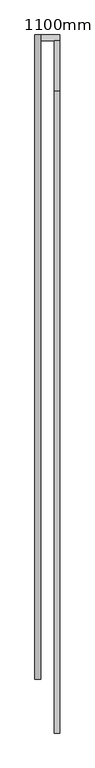
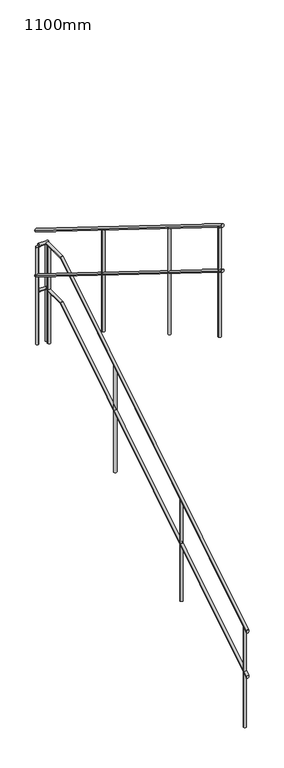
"""IFC4 building model written with IfcOpenShell, lengths in millimetres: railing geometry, 1100mm."""

from ifc_helpers import new_model, si_unit, point, frame, frame_2d, origin, place, context, project, spatial, circle_curve, ellipse_curve, trimmed, segment, composite_curve, outline, extrude, source, transform, mapped, element, save
from ifc_brep_helpers import plane_surface, cylinder_surface, advanced_brep


def railing_1100mm_37236d89(model_context):
    return source(origin(), model_context, "Body", "SolidModel", [
        advanced_brep(
        [(11540.5052251, 14699.5208589, 456.3396197), (11510.5052251, 14699.5208589, 456.3396197), (11540.5052251, 18324.9208589, 2547.0), (11510.5052251, 18324.9208589, 2547.0), (11540.5052251, 18063.8019306, 2547.0), (11510.5052251, 18063.8019306, 2547.0)],
        [
            (0, 1, ellipse_curve(frame((11525.5052251, 14699.5208589, 456.3396197), z_axis=(0.0, -1.0, 0.0), x_axis=(0.0, 0.0, -1.0)), 17.6603803, 15.0)),
            (1, 0, ellipse_curve(frame((11525.5052251, 14699.5208589, 456.3396197), z_axis=(0.0, -1.0, 0.0), x_axis=(0.0, 0.0, -1.0)), 17.6603803, 15.0)),
            (2, 3, circle_curve(frame((11525.5052251, 18324.9208589, 2547.0), z_axis=(0.0, 1.0, 0.0), x_axis=(-1.0, 0.0, 0.0)), 15.0)),
            (3, 2, circle_curve(frame((11525.5052251, 18324.9208589, 2547.0), z_axis=(0.0, 1.0, 0.0), x_axis=(-1.0, 0.0, 0.0)), 15.0)),
            (0, 4),
            (4, 5, ellipse_curve(frame((11525.5052251, 18063.8019306, 2547.0), z_axis=(0.0, -0.9616025257983003, -0.2744459552959912), x_axis=(0.0, 0.2744459552959914, -0.9616025257983002)), 15.5989607, 15.0)),
            (5, 1),
            (5, 4, ellipse_curve(frame((11525.5052251, 18063.8019306, 2547.0), z_axis=(0.0, -0.9616025257983003, -0.2744459552959912), x_axis=(0.0, 0.2744459552959914, -0.9616025257983002)), 15.5989607, 15.0)),
            (4, 2),
            (3, 5),
        ],
        [
            plane_surface(frame((11525.5052251, 14699.5208589, 474.0), z_axis=(0.0, -1.0, 0.0), x_axis=(0.0, 0.0, 1.0))),
            plane_surface(frame((11525.5052251, 18324.9208589, 2562.0), z_axis=(0.0, 1.0, 0.0), x_axis=(0.0, 0.0, 1.0))),
            cylinder_surface(frame((11525.5052251, 14707.4380966, 461.2596175), z_axis=(0.0, -0.8493588352433417, -0.5278158476155052), x_axis=(-1.0, 0.0, 0.0)), 15.0),
            cylinder_surface(frame((11525.5052251, 18059.5208589, 2547.0), z_axis=(0.0, -1.0, 0.0), x_axis=(-1.0, 0.0, 0.0)), 15.0),
        ],
        [
            (0, [[1, 2]]),
            (1, [[3, 4]]),
            (2, [[-1, 5, 6, 7]]),
            (2, [[-2, -7, 8, -5]]),
            (3, [[-6, 9, -4, 10]]),
            (3, [[-8, -10, -3, -9]]),
        ],
    ),
        advanced_brep(
        [(11540.5052251, 18354.9208589, 2547.0), (11540.5052251, 18324.9208589, 2547.0), (11439.7052251, 18354.9208589, 2547.0), (11439.7052251, 18324.9208589, 2547.0)],
        [
            (0, 1, circle_curve(frame((11540.5052251, 18339.9208589, 2547.0), z_axis=(1.0, 0.0, 0.0), x_axis=(0.0, -1.0, 0.0)), 15.0)),
            (1, 0, circle_curve(frame((11540.5052251, 18339.9208589, 2547.0), z_axis=(1.0, 0.0, 0.0), x_axis=(0.0, -1.0, 0.0)), 15.0)),
            (2, 3, circle_curve(frame((11439.7052251, 18339.9208589, 2547.0), z_axis=(-1.0, 0.0, 0.0), x_axis=(0.0, -1.0, 0.0)), 15.0)),
            (3, 2, circle_curve(frame((11439.7052251, 18339.9208589, 2547.0), z_axis=(-1.0, 0.0, 0.0), x_axis=(0.0, -1.0, 0.0)), 15.0)),
            (0, 2),
            (3, 1),
        ],
        [
            plane_surface(frame((11540.5052251, 18339.9208589, 2562.0), z_axis=(1.0, 0.0, 0.0), x_axis=(0.0, -1.0, 0.0))),
            plane_surface(frame((11439.7052251, 18339.9208589, 2562.0), z_axis=(-1.0, 0.0, 0.0), x_axis=(0.0, -1.0, 0.0))),
            cylinder_surface(frame((11540.5052251, 18339.9208589, 2547.0), z_axis=(1.0, 0.0, 0.0), x_axis=(0.0, -1.0, 0.0)), 15.0),
        ],
        [
            (0, [[1, 2]]),
            (1, [[3, 4]]),
            (2, [[-1, 5, -4, 6]]),
            (2, [[-2, -6, -3, -5]]),
        ],
    ),
        advanced_brep(
        [(11409.7052251, 18354.9208589, 2708.7696197), (11439.7052251, 18354.9208589, 2708.7696197), (11409.7052251, 14979.5208589, 4806.3396197), (11439.7052251, 14979.5208589, 4806.3396197)],
        [
            (0, 1, ellipse_curve(frame((11424.7052251, 18354.9208589, 2708.7696197), z_axis=(0.0, 1.0, 0.0), x_axis=(0.0, 0.0, -1.0)), 17.6603803, 15.0)),
            (1, 0, ellipse_curve(frame((11424.7052251, 18354.9208589, 2708.7696197), z_axis=(0.0, 1.0, 0.0), x_axis=(0.0, 0.0, -1.0)), 17.6603803, 15.0)),
            (2, 3, ellipse_curve(frame((11424.7052251, 14979.5208589, 4806.3396197), z_axis=(0.0, -1.0, 0.0), x_axis=(0.0, 0.0, -1.0)), 17.6603803, 15.0)),
            (3, 2, ellipse_curve(frame((11424.7052251, 14979.5208589, 4806.3396197), z_axis=(0.0, -1.0, 0.0), x_axis=(0.0, 0.0, -1.0)), 17.6603803, 15.0)),
            (0, 2),
            (3, 1),
        ],
        [
            plane_surface(frame((11424.7052251, 18354.9208589, 2726.43), z_axis=(0.0, 1.0, 0.0), x_axis=(0.0, 0.0, -1.0))),
            plane_surface(frame((11424.7052251, 14979.5208589, 4824.0), z_axis=(0.0, -1.0, 0.0), x_axis=(0.0, 0.0, -1.0))),
            cylinder_surface(frame((11424.7052251, 18347.0036212, 2713.6896175), z_axis=(0.0, 0.8493588352433417, -0.5278158476155052), x_axis=(1.0, 0.0, 0.0)), 15.0),
        ],
        [
            (0, [[1, 2]]),
            (1, [[3, 4]]),
            (2, [[-1, 5, -4, 6]]),
            (2, [[-2, -6, -3, -5]]),
        ],
    ),
        advanced_brep(
        [(11540.5052251, 14699.5208589, 956.3396197), (11510.5052251, 14699.5208589, 956.3396197), (11540.5052251, 18063.8019306, 3047.0), (11510.5052251, 18063.8019306, 3047.0), (11540.5052251, 18324.9208589, 3047.0), (11510.5052251, 18324.9208589, 3047.0)],
        [
            (0, 1, ellipse_curve(frame((11525.5052251, 14699.5208589, 956.3396197), z_axis=(0.0, -1.0, 0.0), x_axis=(0.0, 0.0, -1.0)), 17.6603803, 15.0)),
            (1, 0, ellipse_curve(frame((11525.5052251, 14699.5208589, 956.3396197), z_axis=(0.0, -1.0, 0.0), x_axis=(0.0, 0.0, -1.0)), 17.6603803, 15.0)),
            (0, 2),
            (2, 3, ellipse_curve(frame((11525.5052251, 18063.8019306, 3047.0), z_axis=(0.0, -0.9616025257983003, -0.2744459552959912), x_axis=(0.0, 0.2744459552959914, -0.9616025257983002)), 15.5989607, 15.0)),
            (3, 1),
            (3, 2, ellipse_curve(frame((11525.5052251, 18063.8019306, 3047.0), z_axis=(0.0, -0.9616025257983003, -0.2744459552959912), x_axis=(0.0, 0.2744459552959914, -0.9616025257983002)), 15.5989607, 15.0)),
            (4, 5, circle_curve(frame((11525.5052251, 18324.9208589, 3047.0), z_axis=(0.0, 1.0, 0.0), x_axis=(-1.0, 0.0, 0.0)), 15.0)),
            (5, 4, circle_curve(frame((11525.5052251, 18324.9208589, 3047.0), z_axis=(0.0, 1.0, 0.0), x_axis=(-1.0, 0.0, 0.0)), 15.0)),
            (2, 4),
            (5, 3),
        ],
        [
            plane_surface(frame((11525.5052251, 14699.5208589, 974.0), z_axis=(0.0, -1.0, 0.0), x_axis=(0.0, 0.0, 1.0))),
            cylinder_surface(frame((11525.5052251, 14707.4380966, 961.2596175), z_axis=(0.0, -0.8493588352433417, -0.5278158476155052), x_axis=(-1.0, 0.0, 0.0)), 15.0),
            plane_surface(frame((11525.5052251, 18324.9208589, 3062.0), z_axis=(0.0, 1.0, 0.0), x_axis=(0.0, 0.0, 1.0))),
            cylinder_surface(frame((11525.5052251, 18059.5208589, 3047.0), z_axis=(0.0, -1.0, 0.0), x_axis=(-1.0, 0.0, 0.0)), 15.0),
        ],
        [
            (0, [[1, 2]]),
            (1, [[-1, 3, 4, 5]]),
            (1, [[-2, -5, 6, -3]]),
            (2, [[7, 8]]),
            (3, [[-4, 9, -8, 10]]),
            (3, [[-6, -10, -7, -9]]),
        ],
    ),
        advanced_brep(
        [(11540.5052251, 18354.9208589, 3047.0), (11540.5052251, 18324.9208589, 3047.0), (11439.7052251, 18354.9208589, 3047.0), (11439.7052251, 18324.9208589, 3047.0)],
        [
            (0, 1, circle_curve(frame((11540.5052251, 18339.9208589, 3047.0), z_axis=(1.0, 0.0, 0.0), x_axis=(0.0, -1.0, 0.0)), 15.0)),
            (1, 0, circle_curve(frame((11540.5052251, 18339.9208589, 3047.0), z_axis=(1.0, 0.0, 0.0), x_axis=(0.0, -1.0, 0.0)), 15.0)),
            (2, 3, circle_curve(frame((11439.7052251, 18339.9208589, 3047.0), z_axis=(-1.0, 0.0, 0.0), x_axis=(0.0, -1.0, 0.0)), 15.0)),
            (3, 2, circle_curve(frame((11439.7052251, 18339.9208589, 3047.0), z_axis=(-1.0, 0.0, 0.0), x_axis=(0.0, -1.0, 0.0)), 15.0)),
            (0, 2),
            (3, 1),
        ],
        [
            plane_surface(frame((11540.5052251, 18339.9208589, 3062.0), z_axis=(1.0, 0.0, 0.0), x_axis=(0.0, -1.0, 0.0))),
            plane_surface(frame((11439.7052251, 18339.9208589, 3062.0), z_axis=(-1.0, 0.0, 0.0), x_axis=(0.0, -1.0, 0.0))),
            cylinder_surface(frame((11540.5052251, 18339.9208589, 3047.0), z_axis=(1.0, 0.0, 0.0), x_axis=(0.0, -1.0, 0.0)), 15.0),
        ],
        [
            (0, [[1, 2]]),
            (1, [[3, 4]]),
            (2, [[-1, 5, -4, 6]]),
            (2, [[-2, -6, -3, -5]]),
        ],
    ),
        advanced_brep(
        [(11409.7052251, 18354.9208589, 3208.7696197), (11439.7052251, 18354.9208589, 3208.7696197), (11409.7052251, 14979.5208589, 5306.3396197), (11439.7052251, 14979.5208589, 5306.3396197)],
        [
            (0, 1, ellipse_curve(frame((11424.7052251, 18354.9208589, 3208.7696197), z_axis=(0.0, 1.0, 0.0), x_axis=(0.0, 0.0, -1.0)), 17.6603803, 15.0)),
            (1, 0, ellipse_curve(frame((11424.7052251, 18354.9208589, 3208.7696197), z_axis=(0.0, 1.0, 0.0), x_axis=(0.0, 0.0, -1.0)), 17.6603803, 15.0)),
            (2, 3, ellipse_curve(frame((11424.7052251, 14979.5208589, 5306.3396197), z_axis=(0.0, -1.0, 0.0), x_axis=(0.0, 0.0, -1.0)), 17.6603803, 15.0)),
            (3, 2, ellipse_curve(frame((11424.7052251, 14979.5208589, 5306.3396197), z_axis=(0.0, -1.0, 0.0), x_axis=(0.0, 0.0, -1.0)), 17.6603803, 15.0)),
            (0, 2),
            (3, 1),
        ],
        [
            plane_surface(frame((11424.7052251, 18354.9208589, 3226.43), z_axis=(0.0, 1.0, 0.0), x_axis=(0.0, 0.0, -1.0))),
            plane_surface(frame((11424.7052251, 14979.5208589, 5324.0), z_axis=(0.0, -1.0, 0.0), x_axis=(0.0, 0.0, -1.0))),
            cylinder_surface(frame((11424.7052251, 18347.0036212, 3213.6896175), z_axis=(0.0, 0.8493588352433417, -0.5278158476155052), x_axis=(1.0, 0.0, 0.0)), 15.0),
        ],
        [
            (0, [[1, 2]]),
            (1, [[3, 4]]),
            (2, [[-1, 5, -4, 6]]),
            (2, [[-2, -6, -3, -5]]),
        ],
    ),
        extrude(outline(composite_curve([segment(trimmed(circle_curve(frame_2d((11424.7052251, 15939.9208589)), 15.0), [point((11439.7052251, 15939.9208589))], [point((11409.7052251, 15939.9208589))], False, "CARTESIAN"), True, "CONTINUOUS"), segment(trimmed(circle_curve(frame_2d((11424.7052251, 15939.9208589)), 15.0), [point((11409.7052251, 15939.9208589))], [point((11439.7052251, 15939.9208589))], False, "CARTESIAN"), True, "CONTINUOUS")], self_intersect=False)), frame((0.0, 0.0, 3528.0), z_axis=(0.0, 0.0, 1.0), x_axis=(1.0, 0.0, 0.0)), (0.0, 0.0, 1.0), 1169.18),
        extrude(outline(composite_curve([segment(trimmed(circle_curve(frame_2d((11424.7052251, 17139.9208589)), 15.0), [point((11439.7052251, 17139.9208589))], [point((11409.7052251, 17139.9208589))], False, "CARTESIAN"), True, "CONTINUOUS"), segment(trimmed(circle_curve(frame_2d((11424.7052251, 17139.9208589)), 15.0), [point((11409.7052251, 17139.9208589))], [point((11439.7052251, 17139.9208589))], False, "CARTESIAN"), True, "CONTINUOUS")], self_intersect=False)), frame((0.0, 0.0, 2832.0), z_axis=(0.0, 0.0, 1.0), x_axis=(1.0, 0.0, 0.0)), (0.0, 0.0, 1.0), 1119.4657143),
        extrude(outline(composite_curve([segment(trimmed(circle_curve(frame_2d((11525.5052251, 18299.5208589)), 15.0), [point((11510.5052251, 18299.5208589))], [point((11540.5052251, 18299.5208589))], False, "CARTESIAN"), True, "CONTINUOUS"), segment(trimmed(circle_curve(frame_2d((11525.5052251, 18299.5208589)), 15.0), [point((11540.5052251, 18299.5208589))], [point((11510.5052251, 18299.5208589))], False, "CARTESIAN"), True, "CONTINUOUS")], self_intersect=False)), frame((0.0, 0.0, 1962.0), z_axis=(0.0, 0.0, 1.0), x_axis=(1.0, 0.0, 0.0)), (0.0, 0.0, 1.0), 1070.0),
        extrude(outline(composite_curve([segment(trimmed(circle_curve(frame_2d((11525.5052251, 17099.5208589)), 15.0), [point((11510.5052251, 17099.5208589))], [point((11540.5052251, 17099.5208589))], False, "CARTESIAN"), True, "CONTINUOUS"), segment(trimmed(circle_curve(frame_2d((11525.5052251, 17099.5208589)), 15.0), [point((11540.5052251, 17099.5208589))], [point((11510.5052251, 17099.5208589))], False, "CARTESIAN"), True, "CONTINUOUS")], self_intersect=False)), frame((0.0, 0.0, 1266.0), z_axis=(0.0, 0.0, 1.0), x_axis=(1.0, 0.0, 0.0)), (0.0, 0.0, 1.0), 1169.4285714),
        extrude(outline(composite_curve([segment(trimmed(circle_curve(frame_2d((11525.5052251, 15899.5208589)), 15.0), [point((11510.5052251, 15899.5208589))], [point((11540.5052251, 15899.5208589))], False, "CARTESIAN"), True, "CONTINUOUS"), segment(trimmed(circle_curve(frame_2d((11525.5052251, 15899.5208589)), 15.0), [point((11540.5052251, 15899.5208589))], [point((11510.5052251, 15899.5208589))], False, "CARTESIAN"), True, "CONTINUOUS")], self_intersect=False)), frame((0.0, 0.0, 570.0), z_axis=(0.0, 0.0, 1.0), x_axis=(1.0, 0.0, 0.0)), (0.0, 0.0, 1.0), 1119.7142857),
        extrude(outline(composite_curve([segment(trimmed(circle_curve(frame_2d((11424.7052251, 18339.9208589)), 15.0), [point((11424.7052251, 18324.9208589))], [point((11424.7052251, 18354.9208589))], False, "CARTESIAN"), True, "CONTINUOUS"), segment(trimmed(circle_curve(frame_2d((11424.7052251, 18339.9208589)), 15.0), [point((11424.7052251, 18354.9208589))], [point((11424.7052251, 18324.9208589))], False, "CARTESIAN"), True, "CONTINUOUS")], self_intersect=False)), frame((0.0, 0.0, 1962.0), z_axis=(0.0, 0.0, 1.0), x_axis=(1.0, 0.0, 0.0)), (0.0, 0.0, 1.0), 1070.0),
        extrude(outline(composite_curve([segment(trimmed(circle_curve(frame_2d((11525.5052251, 18339.9208589)), 15.0), [point((11510.5052251, 18339.9208589))], [point((11540.5052251, 18339.9208589))], False, "CARTESIAN"), True, "CONTINUOUS"), segment(trimmed(circle_curve(frame_2d((11525.5052251, 18339.9208589)), 15.0), [point((11540.5052251, 18339.9208589))], [point((11510.5052251, 18339.9208589))], False, "CARTESIAN"), True, "CONTINUOUS")], self_intersect=False)), frame((0.0, 0.0, 1962.0), z_axis=(0.0, 0.0, 1.0), x_axis=(1.0, 0.0, 0.0)), (0.0, 0.0, 1.0), 1070.0),
        extrude(outline(composite_curve([segment(trimmed(circle_curve(frame_2d((11424.7052251, 15029.5208589)), 15.0), [point((11439.7052251, 15029.5208589))], [point((11409.7052251, 15029.5208589))], False, "CARTESIAN"), True, "CONTINUOUS"), segment(trimmed(circle_curve(frame_2d((11424.7052251, 15029.5208589)), 15.0), [point((11409.7052251, 15029.5208589))], [point((11439.7052251, 15029.5208589))], False, "CARTESIAN"), True, "CONTINUOUS")], self_intersect=False)), frame((0.0, 0.0, 4050.0), z_axis=(0.0, 0.0, 1.0), x_axis=(1.0, 0.0, 0.0)), (0.0, 0.0, 1.0), 1212.9285714),
        extrude(outline(composite_curve([segment(trimmed(circle_curve(frame_2d((11525.5052251, 14749.5208589)), 15.0), [point((11510.5052251, 14749.5208589))], [point((11540.5052251, 14749.5208589))], False, "CARTESIAN"), True, "CONTINUOUS"), segment(trimmed(circle_curve(frame_2d((11525.5052251, 14749.5208589)), 15.0), [point((11540.5052251, 14749.5208589))], [point((11510.5052251, 14749.5208589))], False, "CARTESIAN"), True, "CONTINUOUS")], self_intersect=False)), frame((0.0, 0.0, -126.0), z_axis=(0.0, 0.0, 1.0), x_axis=(1.0, 0.0, 0.0)), (0.0, 0.0, 1.0), 1101.0714286),
    ])


if __name__ == "__main__":
    model = new_model("IFC4")
    model_context = context("Model", 3, world=origin())
    ifc_project = project(units=[si_unit("LENGTHUNIT", "METRE", prefix="MILLI")], contexts=[model_context])
    site = spatial("IfcSite", under=ifc_project)
    building = spatial("IfcBuilding", under=site)
    placement = place(None, origin())
    railing_1100mm_shape = railing_1100mm_37236d89(model_context)
    element("IfcRailing", 1, ObjectType="1100mm", at=placement, inside=building, context=model_context, shape_type="MappedRepresentation", body=[
        mapped(railing_1100mm_shape, transform((0.0, 0.0, 0.0), x_axis=(1.0, 0.0, 0.0), y_axis=(0.0, 1.0, 0.0), z_axis=(0.0, 0.0, 1.0))),
    ])
    save(model, "model.ifc")
